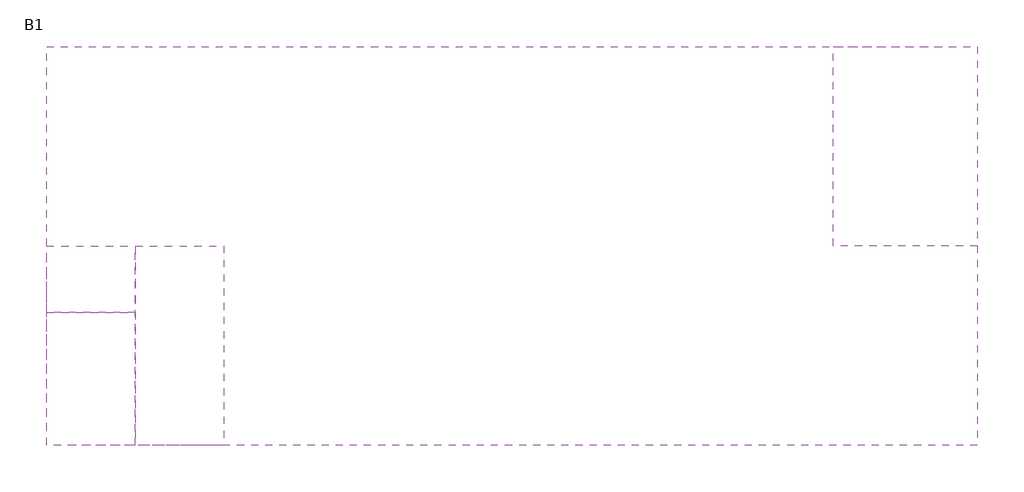
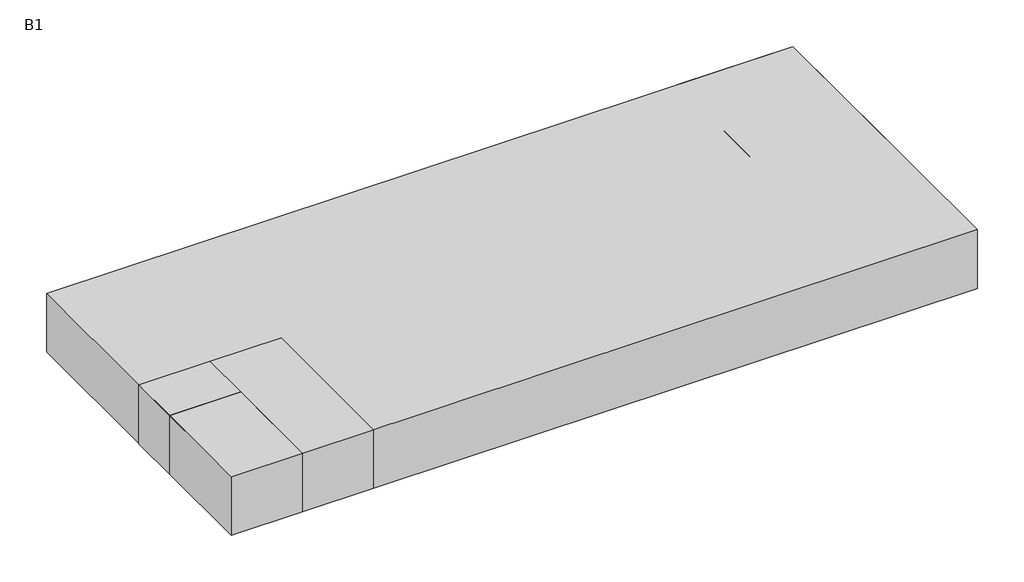
# One storey: 5 proxies.
"""IFC4 building model written with IfcOpenShell, lengths in millimetres."""

import ifcopenshell
import ifcopenshell.guid

model = None  # the IFC model being written
_history = None  # IfcOwnerHistory: only IFC2X3 demands one
_inside = {}  # id of a spatial element -> (the spatial element, [elements in it])
_under = {}  # id of a project, library or spatial element -> (it, [spatial elements below it])
_declared = {}  # id of a project -> (the project, [libraries it declares])
_typed = {}  # id of a type object -> (the type object, [elements of that type])
_made_of = {}  # id of a material, layer set ... -> (it, [elements and type objects made of it])


def new_model(schema):
    """Start an empty IFC model of exactly this schema.

    Asked for "IFC4X3", IfcOpenShell would pick the latest addendum, in which some entities
    have other attributes; the version numbers below select the first issue.
    IFC2X3 requires an IfcOwnerHistory on every rooted entity: one is made here for all.
    """
    global model, _history
    if schema == "IFC4X3":
        model = ifcopenshell.file(schema_version=(4, 3, 0, 0))
    else:
        model = ifcopenshell.file(schema=schema)
    _inside.clear()
    _under.clear()
    _declared.clear()
    _typed.clear()
    _made_of.clear()
    _history = None
    if model.schema == "IFC2X3":
        org = make("IfcOrganization", Name="unknown")
        user = make(
            "IfcPersonAndOrganization",
            ThePerson=make("IfcPerson", FamilyName="unknown"),
            TheOrganization=org,
        )
        app = make(
            "IfcApplication",
            ApplicationDeveloper=org,
            Version="unknown",
            ApplicationFullName="unknown",
            ApplicationIdentifier="unknown",
        )
        _history = make(
            "IfcOwnerHistory",
            OwningUser=user,
            OwningApplication=app,
            ChangeAction="ADDED",
            CreationDate=0,
        )
    return model


def make(cls, **values):
    """One entity of the class cls with the attributes given. An attribute that is None is left unset."""
    return model.create_entity(
        cls, **{name: value for name, value in values.items() if value is not None}
    )


def rooted(cls, **values):
    """An entity with a GlobalId (a new one), such as an element, a storey or a relation."""
    return make(cls, GlobalId=ifcopenshell.guid.new(), OwnerHistory=_history, **values)


def si_unit(unit_type, name, prefix=None):
    """IfcSIUnit, for example si_unit("LENGTHUNIT", "METRE", prefix="MILLI")."""
    return make("IfcSIUnit", UnitType=unit_type, Prefix=prefix, Name=name)


def assignment(units):
    """IfcUnitAssignment: the units of a project."""
    return None if units is None else make("IfcUnitAssignment", Units=units)


def point(xyz):
    """IfcCartesianPoint."""
    return None if xyz is None else make("IfcCartesianPoint", Coordinates=xyz)


def direction(xyz):
    """IfcDirection."""
    return None if xyz is None else make("IfcDirection", DirectionRatios=xyz)


def frame(location, z_axis=None, x_axis=None):
    """IfcAxis2Placement3D, a coordinate frame: its origin and axes. An axis left out is left unset."""
    return make(
        "IfcAxis2Placement3D",
        Location=point(location),
        Axis=direction(z_axis),
        RefDirection=direction(x_axis),
    )


def origin():
    """The frame at (0, 0, 0) with its axes left unset."""
    return frame((0.0, 0.0, 0.0))


def origin_with_axes():
    """The frame at (0, 0, 0) with the z axis (0, 0, 1) and the x axis (1, 0, 0) written out."""
    return frame((0.0, 0.0, 0.0), z_axis=(0.0, 0.0, 1.0), x_axis=(1.0, 0.0, 0.0))


def place(relative_to, where):
    """IfcLocalPlacement: puts the frame where relative to a parent placement (None: the world)."""
    return make(
        "IfcLocalPlacement", PlacementRelTo=relative_to, RelativePlacement=where
    )


def context(
    kind, dimensions, precision=None, world=None, true_north=None, identifier=None
):
    """IfcGeometricRepresentationContext, for example the 3D "Model" context."""
    return make(
        "IfcGeometricRepresentationContext",
        ContextIdentifier=identifier,
        ContextType=kind,
        CoordinateSpaceDimension=dimensions,
        Precision=precision,
        WorldCoordinateSystem=world,
        TrueNorth=true_north,
    )


def project(units=None, contexts=None):
    """IfcProject with its units and contexts."""
    return rooted(
        "IfcProject",
        Name="project",
        RepresentationContexts=contexts,
        UnitsInContext=assignment(units),
    )


def spatial(cls, under=None, at=None, **own):
    """A site, building, storey or space (cls), placed at a placement, below another one or the project."""
    s = rooted(cls, ObjectPlacement=at, **own)
    if under is not None:
        _under.setdefault(under.id(), (under, []))[1].append(s)
    return s


def polyline(points):
    """IfcPolyline through the points."""
    return make("IfcPolyline", Points=[point(p) for p in points])


def outline(outer, holes=None, kind="AREA"):
    """IfcArbitraryClosedProfileDef: a profile drawn as a closed curve; with holes, ...WithVoids."""
    if holes is None:
        return make("IfcArbitraryClosedProfileDef", ProfileType=kind, OuterCurve=outer)
    return make(
        "IfcArbitraryProfileDefWithVoids",
        ProfileType=kind,
        OuterCurve=outer,
        InnerCurves=holes,
    )


def extrude(swept, where, along, depth):
    """IfcExtrudedAreaSolid: the profile swept, set in the frame where, extruded along a direction by depth."""
    return make(
        "IfcExtrudedAreaSolid",
        SweptArea=swept,
        Position=where,
        ExtrudedDirection=direction(along),
        Depth=depth,
    )


def shape(context_of_items, identifier, shape_type, items):
    """IfcShapeRepresentation: the items that make up one representation, for example the "Body"."""
    return make(
        "IfcShapeRepresentation",
        ContextOfItems=context_of_items,
        RepresentationIdentifier=identifier,
        RepresentationType=shape_type,
        Items=items,
    )


def source(mapping_origin, context_of_items, identifier, shape_type, items):
    """IfcRepresentationMap: a shape defined once, which mapped items show again and again."""
    return make(
        "IfcRepresentationMap",
        MappingOrigin=mapping_origin,
        MappedRepresentation=shape(context_of_items, identifier, shape_type, items),
    )


def transform(
    local_origin,
    x_axis=None,
    y_axis=None,
    z_axis=None,
    scale=None,
    scale2=None,
    scale3=None,
    uniform=True,
):
    """IfcCartesianTransformationOperator3D, or its non-uniform kind. x_axis, y_axis, z_axis: its Axis1, 2, 3."""
    if uniform:
        return make(
            "IfcCartesianTransformationOperator3D",
            Axis1=direction(x_axis),
            Axis2=direction(y_axis),
            LocalOrigin=point(local_origin),
            Scale=scale,
            Axis3=direction(z_axis),
        )
    return make(
        "IfcCartesianTransformationOperator3DnonUniform",
        Axis1=direction(x_axis),
        Axis2=direction(y_axis),
        LocalOrigin=point(local_origin),
        Scale=scale,
        Axis3=direction(z_axis),
        Scale2=scale2,
        Scale3=scale3,
    )


def mapped(mapping_source, mapping_target):
    """IfcMappedItem: shows the shape of a source again, moved by a transform."""
    return make(
        "IfcMappedItem", MappingSource=mapping_source, MappingTarget=mapping_target
    )


def made_of(thing, what):
    """Note that an element or type object is made of a material, layer set ...; save() writes the relation."""
    if what is not None:
        _made_of.setdefault(what.id(), (what, []))[1].append(thing)
    return thing


def element(
    cls,
    number,
    at=None,
    inside=None,
    cuts=None,
    type_object=None,
    material=None,
    context=None,
    identifier="Body",
    shape_type=None,
    held_by="IfcProductDefinitionShape",
    body=None,
    shapes=None,
    **own,
):
    """One element of the class cls, such as IfcWall. Its Tag is "e" and its number.

    at: its placement. inside: the storey or other place that contains it. cuts: it is an
    opening in that element (IfcRelVoidsElement). A single representation is given by context,
    identifier, shape_type and body (its items); several are given by shapes. held_by: the class
    of the entity that holds the representations. save() writes the other relations.
    """
    e = rooted(cls, Tag="e%d" % number, ObjectPlacement=at, **own)
    if body is not None:
        shapes = [shape(context, identifier, shape_type, body)]
    if shapes is not None:
        e.Representation = make(held_by, Representations=shapes)
    if inside is not None:
        _inside.setdefault(inside.id(), (inside, []))[1].append(e)
    if cuts is not None:
        rooted(
            "IfcRelVoidsElement", RelatingBuildingElement=cuts, RelatedOpeningElement=e
        )
    if type_object is not None:
        _typed.setdefault(type_object.id(), (type_object, []))[1].append(e)
    return made_of(e, material)


def aggregate(whole, parts):
    """IfcRelAggregates: a whole, such as a stair, and the parts it consists of."""
    return rooted("IfcRelAggregates", RelatingObject=whole, RelatedObjects=parts)


def save(model, path):
    """Write the relations noted so far, then the file.

    IfcRelAggregates (storeys below a building ...), IfcRelContainedInSpatialStructure (elements
    in a storey), IfcRelDefinesByType, IfcRelAssociatesMaterial and IfcRelDeclares: one each for
    every whole, place, type object, material and project.
    """
    for whole, parts in _under.values():
        aggregate(whole, parts)
    for where, things in _inside.values():
        rooted(
            "IfcRelContainedInSpatialStructure",
            RelatedElements=things,
            RelatingStructure=where,
        )
    for kind, things in _typed.values():
        rooted("IfcRelDefinesByType", RelatedObjects=things, RelatingType=kind)
    for what, things in _made_of.values():
        rooted("IfcRelAssociatesMaterial", RelatedObjects=things, RelatingMaterial=what)
    for by, libraries in _declared.values():
        rooted("IfcRelDeclares", RelatingContext=by, RelatedDefinitions=libraries)
    model.write(path)


def generic_models_bb515c93(model_context):
    return source(origin(), model_context, "Body", "SweptSolid", [
        extrude(outline(polyline([(9000.0, 21000.0), (9000.0, -21000.0), (-9000.0, -21000.0), (-9000.0, 21000.0), (9000.0, 21000.0)])), origin_with_axes(), (0.0, 0.0, 1.0), 3500.0),
    ])


def generic_models_5926095e(model_context):
    return source(origin(), model_context, "Body", "SweptSolid", [
        extrude(outline(polyline([(3250.0, 4500.0), (3250.0, -4500.0), (-3250.0, -4500.0), (-3250.0, 4500.0), (3250.0, 4500.0)])), origin_with_axes(), (0.0, 0.0, 1.0), 3500.0),
    ])


def generic_models_0b067365(model_context):
    return source(origin(), model_context, "Body", "SweptSolid", [
        extrude(outline(polyline([(2000.0, 4500.0), (2000.0, -4500.0), (-2000.0, -4500.0), (-2000.0, 4500.0), (2000.0, 4500.0)])), origin_with_axes(), (0.0, 0.0, 1.0), 3500.0),
    ])


def generic_models_4c644d41(model_context):
    return source(origin(), model_context, "Body", "SweptSolid", [
        extrude(outline(polyline([(2000.0, 1500.0), (2000.0, -1500.0), (-2000.0, -1500.0), (-2000.0, 1500.0), (2000.0, 1500.0)])), origin_with_axes(), (0.0, 0.0, 1.0), 3500.0),
    ])


def generic_models_c89eb543(model_context):
    return source(origin(), model_context, "Body", "SweptSolid", [
        extrude(outline(polyline([(2000.0, 3000.0), (2000.0, -3000.0), (-2000.0, -3000.0), (-2000.0, 3000.0), (2000.0, 3000.0)])), origin_with_axes(), (0.0, 0.0, 1.0), 3500.0),
    ])


model = new_model("IFC4")

# Units and contexts
model_context = context("Model", 3, world=origin())
ifc_project = project(units=[si_unit("LENGTHUNIT", "METRE", prefix="MILLI")], contexts=[model_context])

# Site, building, storey
site = spatial("IfcSite", under=ifc_project)
building = spatial("IfcBuilding", under=site)
storey = spatial("IfcBuildingStorey", under=building, Name="B1", Elevation=-4000.0)

# Proxies
placement = place(None, origin())
generic_models_shape = generic_models_bb515c93(model_context)
element("IfcBuildingElementProxy", 1, Name="Space Planning Box_hec : Space Planning Box_hec", ObjectType="Space Planning Box_hec : Space Planning Box_hec", at=placement, inside=storey, context=model_context, shape_type="MappedRepresentation", body=[
    mapped(generic_models_shape, transform((66459.6521483, 172923.8614395, 0.0), x_axis=(0.0, -1.0, 0.0), y_axis=(1.0, 0.0, 0.0), z_axis=(0.0, 0.0, 1.0))),
])
generic_models_2_shape = generic_models_5926095e(model_context)
element("IfcBuildingElementProxy", 2, Name="Space Planning Box_hec : Space Planning Box_hec", ObjectType="Space Planning Box_hec : Space Planning Box_hec", at=placement, inside=storey, context=model_context, shape_type="MappedRepresentation", body=[
    mapped(generic_models_2_shape, transform((84209.6521483, 177423.8614395, 0.0), x_axis=(1.0, 0.0, 0.0), y_axis=(0.0, 1.0, 0.0), z_axis=(0.0, 0.0, 1.0))),
])
generic_models_3_shape = generic_models_0b067365(model_context)
element("IfcBuildingElementProxy", 3, Name="Space Planning Box_hec : Space Planning Box_hec", ObjectType="Space Planning Box_hec : Space Planning Box_hec", at=placement, inside=storey, context=model_context, shape_type="MappedRepresentation", body=[
    mapped(generic_models_3_shape, transform((51459.6521483, 168423.8614395, 0.0), x_axis=(1.0, 0.0, 0.0), y_axis=(0.0, 1.0, 0.0), z_axis=(0.0, 0.0, 1.0))),
])
generic_models_4_shape = generic_models_4c644d41(model_context)
element("IfcBuildingElementProxy", 4, Name="Space Planning Box_hec : Space Planning Box_hec", ObjectType="Space Planning Box_hec : Space Planning Box_hec", at=placement, inside=storey, context=model_context, shape_type="MappedRepresentation", body=[
    mapped(generic_models_4_shape, transform((47459.6521483, 171423.8614395, 0.0), x_axis=(1.0, 0.0, 0.0), y_axis=(0.0, 1.0, 0.0), z_axis=(0.0, 0.0, 1.0))),
])
generic_models_5_shape = generic_models_c89eb543(model_context)
element("IfcBuildingElementProxy", 5, Name="Space Planning Box_hec : Space Planning Box_hec", ObjectType="Space Planning Box_hec : Space Planning Box_hec", at=placement, inside=storey, context=model_context, shape_type="MappedRepresentation", body=[
    mapped(generic_models_5_shape, transform((47459.6521483, 166923.8614395, 0.0), x_axis=(1.0, 0.0, 0.0), y_axis=(0.0, 1.0, 0.0), z_axis=(0.0, 0.0, 1.0))),
])

save(model, "model.ifc")

# Revit data of these elements
# Project information
#   Building Name = "MAIN GATE SECURITY BUILDING"
#   Project Status = "Project Status"
#   Client Name = "현대엔지니어링"
#   Project Address = "서울시 종로구 율곡로 75(계동)"
#   Project Name = "Therma Visayas Energy Project"
#   Project Number = "-"
# Grids (mm)
#   "1": line (45459.652, 190234.526) -> (45459.652, 152139.384)
#   "2": line (53459.652, 190234.526) -> (53459.652, 152139.384)
#   "3": line (61459.652, 190234.526) -> (61459.652, 152139.384)
#   "4": line (69459.652, 190234.526) -> (69459.652, 152139.384)
#   "5": line (77459.652, 190234.526) -> (77459.652, 152139.384)
#   "6": line (87459.652, 190234.526) -> (87459.652, 152139.384)
#   "C": line (39389.066, 181923.861) -> (102402.798, 181923.861)
#   "B": line (39389.066, 172923.861) -> (102402.798, 172923.861)
#   "A": line (39389.066, 163923.861) -> (102402.798, 163923.861)
# Type "Space Planning Box_hec : Space Planning Box_hec"
#   Type Comments = "..."
#   Room Name [instance default] = "?"
#   Interior Finish [instance default] = ""
#   Exterior Finish [instance default] = ""
#   Department [instance default] = ""
#   Assembly Code = "..."
#   Width [instance default] = 1524 mm
#   Program Area [instance default] = 0.00 m²
#   Length [instance default] = 1524 mm
#   Height [instance default] = 1524 mm
#   Area [instance default] = 2.32258 m²
#   Fill Color [instance default] = Cyan
#   Default Elevation = 0
# Element 1 (IfcBuildingElementProxy, "Space Planning Box_hec : Space Planning Box_hec")
#   Room Name = "Cable Room"
#   Interior Finish = "IW5..IW2..N/A,,WK1..N/A,,FL1,,CL1..N/A"
#   Exterior Finish = "N/A..N/A,,EW1..EW2..N/A"
#   Department = "EL"
#   Width = 18000 mm
#   Program Area = 720.00 m²
#   Length = 42000 mm
#   Height = 3500 mm
#   Area = 756.00 m²
#   Fill Color = Orange
#   Phase Created = New Construction
#   Materials on its faces: "Orange"
# Element 2 (IfcBuildingElementProxy, "Space Planning Box_hec : Space Planning Box_hec")
#   Room Name = "Battery Room"
#   Interior Finish = "IW2..N/A..N/A,,N/A..N/A,,FL7,,CL2..N/A"
#   Exterior Finish = "N/A..N/A,,EW2..N/A..N/A"
#   Department = "EL"
#   Width = 6500 mm
#   Program Area = 58.50 m²
#   Length = 9000 mm
#   Height = 3500 mm
#   Area = 58.50 m²
#   Fill Color = Orange
#   Phase Created = New Construction
#   Materials on its faces: "Orange"
# Element 3 (IfcBuildingElementProxy, "Space Planning Box_hec : Space Planning Box_hec")
#   Room Name = "Lobby"
#   Interior Finish = "IW5..N/A..N/A,,WK3..N/A,,FL2,,N/A..N/A"
#   Exterior Finish = "N/A..N/A,,EW2..N/A..N/A"
#   Department = "AR"
#   Width = 4000 mm
#   Program Area = 0.00 m²
#   Length = 9000 mm
#   Height = 3500 mm
#   Area = 36.00 m²
#   Fill Color = Cyan
#   Phase Created = New Construction
#   Materials on its faces: "Cyan"
# Element 4 (IfcBuildingElementProxy, "Space Planning Box_hec : Space Planning Box_hec")
#   Room Name = "Elevator"
#   Interior Finish = "N/A..N/A..N/A,,N/A..N/A,,,,CL3..N/A"
#   Exterior Finish = "N/A..N/A,,EW2..N/A..N/A"
#   Department = "AR"
#   Width = 4000 mm
#   Program Area = 0.00 m²
#   Length = 3000 mm
#   Height = 3500 mm
#   Area = 12.00 m²
#   Fill Color = Cyan
#   Phase Created = New Construction
#   Materials on its faces: "Cyan"
# Element 5 (IfcBuildingElementProxy, "Space Planning Box_hec : Space Planning Box_hec")
#   Room Name = "Stairway"
#   Interior Finish = "IW5..N/A..N/A,,WK3..N/A,,FL2,,CL1..N/A"
#   Exterior Finish = "N/A..N/A,,EW2..N/A..N/A"
#   Department = "PATHV1"
#   Width = 4000 mm
#   Program Area = 36.00 m²
#   Length = 6000 mm
#   Height = 3500 mm
#   Area = 24.00 m²
#   Fill Color = Green
#   Phase Created = New Construction
#   Materials on its faces: "Green"
# Materials
#   "Cyan": class "Generic", colour RGB 0 255 255, transparency 0.2, Cost = 0
#   "Orange": class "Generic", colour RGB 255 165 0, transparency 0.2, Cost = 0
#   "Green": class "Generic", colour RGB 0 128 0, transparency 0.2, Cost = 0
